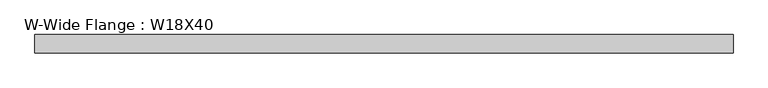
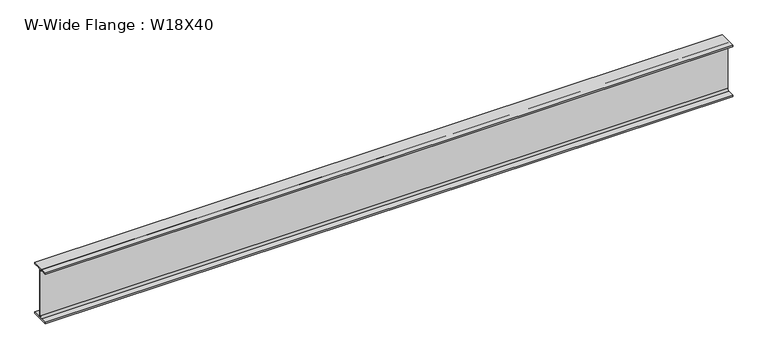
"""IFC4 building model written with IfcOpenShell, lengths in millimetres: beam geometry, W-Wide Flange : W18X40."""

import ifcopenshell
import ifcopenshell.guid

model = None  # the IFC model being written
_history = None  # IfcOwnerHistory: only IFC2X3 demands one
_inside = {}  # id of a spatial element -> (the spatial element, [elements in it])
_under = {}  # id of a project, library or spatial element -> (it, [spatial elements below it])
_declared = {}  # id of a project -> (the project, [libraries it declares])
_typed = {}  # id of a type object -> (the type object, [elements of that type])
_made_of = {}  # id of a material, layer set ... -> (it, [elements and type objects made of it])


def new_model(schema):
    """Start an empty IFC model of exactly this schema.

    Asked for "IFC4X3", IfcOpenShell would pick the latest addendum, in which some entities
    have other attributes; the version numbers below select the first issue.
    IFC2X3 requires an IfcOwnerHistory on every rooted entity: one is made here for all.
    """
    global model, _history
    if schema == "IFC4X3":
        model = ifcopenshell.file(schema_version=(4, 3, 0, 0))
    else:
        model = ifcopenshell.file(schema=schema)
    _inside.clear()
    _under.clear()
    _declared.clear()
    _typed.clear()
    _made_of.clear()
    _history = None
    if model.schema == "IFC2X3":
        org = make("IfcOrganization", Name="unknown")
        user = make(
            "IfcPersonAndOrganization",
            ThePerson=make("IfcPerson", FamilyName="unknown"),
            TheOrganization=org,
        )
        app = make(
            "IfcApplication",
            ApplicationDeveloper=org,
            Version="unknown",
            ApplicationFullName="unknown",
            ApplicationIdentifier="unknown",
        )
        _history = make(
            "IfcOwnerHistory",
            OwningUser=user,
            OwningApplication=app,
            ChangeAction="ADDED",
            CreationDate=0,
        )
    return model


def make(cls, **values):
    """One entity of the class cls with the attributes given. An attribute that is None is left unset."""
    return model.create_entity(
        cls, **{name: value for name, value in values.items() if value is not None}
    )


def rooted(cls, **values):
    """An entity with a GlobalId (a new one), such as an element, a storey or a relation."""
    return make(cls, GlobalId=ifcopenshell.guid.new(), OwnerHistory=_history, **values)


def si_unit(unit_type, name, prefix=None):
    """IfcSIUnit, for example si_unit("LENGTHUNIT", "METRE", prefix="MILLI")."""
    return make("IfcSIUnit", UnitType=unit_type, Prefix=prefix, Name=name)


def assignment(units):
    """IfcUnitAssignment: the units of a project."""
    return None if units is None else make("IfcUnitAssignment", Units=units)


def point(xyz):
    """IfcCartesianPoint."""
    return None if xyz is None else make("IfcCartesianPoint", Coordinates=xyz)


def direction(xyz):
    """IfcDirection."""
    return None if xyz is None else make("IfcDirection", DirectionRatios=xyz)


def frame(location, z_axis=None, x_axis=None):
    """IfcAxis2Placement3D, a coordinate frame: its origin and axes. An axis left out is left unset."""
    return make(
        "IfcAxis2Placement3D",
        Location=point(location),
        Axis=direction(z_axis),
        RefDirection=direction(x_axis),
    )


def frame_2d(location, x_axis=None):
    """IfcAxis2Placement2D, a coordinate frame in the plane: its origin and x axis."""
    return make(
        "IfcAxis2Placement2D", Location=point(location), RefDirection=direction(x_axis)
    )


def origin():
    """The frame at (0, 0, 0) with its axes left unset."""
    return frame((0.0, 0.0, 0.0))


def place(relative_to, where):
    """IfcLocalPlacement: puts the frame where relative to a parent placement (None: the world)."""
    return make(
        "IfcLocalPlacement", PlacementRelTo=relative_to, RelativePlacement=where
    )


def context(
    kind, dimensions, precision=None, world=None, true_north=None, identifier=None
):
    """IfcGeometricRepresentationContext, for example the 3D "Model" context."""
    return make(
        "IfcGeometricRepresentationContext",
        ContextIdentifier=identifier,
        ContextType=kind,
        CoordinateSpaceDimension=dimensions,
        Precision=precision,
        WorldCoordinateSystem=world,
        TrueNorth=true_north,
    )


def project(units=None, contexts=None):
    """IfcProject with its units and contexts."""
    return rooted(
        "IfcProject",
        Name="project",
        RepresentationContexts=contexts,
        UnitsInContext=assignment(units),
    )


def spatial(cls, under=None, at=None, **own):
    """A site, building, storey or space (cls), placed at a placement, below another one or the project."""
    s = rooted(cls, ObjectPlacement=at, **own)
    if under is not None:
        _under.setdefault(under.id(), (under, []))[1].append(s)
    return s


def polyline(points):
    """IfcPolyline through the points."""
    return make("IfcPolyline", Points=[point(p) for p in points])


def circle_curve(where, radius):
    """IfcCircle in the frame where."""
    return make("IfcCircle", Position=where, Radius=radius)


def trimmed(basis, trim1, trim2, sense, master):
    """IfcTrimmedCurve: the piece of a basis curve between two trims."""
    return make(
        "IfcTrimmedCurve",
        BasisCurve=basis,
        Trim1=trim1,
        Trim2=trim2,
        SenseAgreement=sense,
        MasterRepresentation=master,
    )


def segment(curve, same_sense, transition):
    """IfcCompositeCurveSegment."""
    return make(
        "IfcCompositeCurveSegment",
        Transition=transition,
        SameSense=same_sense,
        ParentCurve=curve,
    )


def composite_curve(segments, self_intersect=None):
    """IfcCompositeCurve: segments joined end to end."""
    return make("IfcCompositeCurve", Segments=segments, SelfIntersect=self_intersect)


def outline(outer, holes=None, kind="AREA"):
    """IfcArbitraryClosedProfileDef: a profile drawn as a closed curve; with holes, ...WithVoids."""
    if holes is None:
        return make("IfcArbitraryClosedProfileDef", ProfileType=kind, OuterCurve=outer)
    return make(
        "IfcArbitraryProfileDefWithVoids",
        ProfileType=kind,
        OuterCurve=outer,
        InnerCurves=holes,
    )


def extrude(swept, where, along, depth):
    """IfcExtrudedAreaSolid: the profile swept, set in the frame where, extruded along a direction by depth."""
    return make(
        "IfcExtrudedAreaSolid",
        SweptArea=swept,
        Position=where,
        ExtrudedDirection=direction(along),
        Depth=depth,
    )


def shape(context_of_items, identifier, shape_type, items):
    """IfcShapeRepresentation: the items that make up one representation, for example the "Body"."""
    return make(
        "IfcShapeRepresentation",
        ContextOfItems=context_of_items,
        RepresentationIdentifier=identifier,
        RepresentationType=shape_type,
        Items=items,
    )


def source(mapping_origin, context_of_items, identifier, shape_type, items):
    """IfcRepresentationMap: a shape defined once, which mapped items show again and again."""
    return make(
        "IfcRepresentationMap",
        MappingOrigin=mapping_origin,
        MappedRepresentation=shape(context_of_items, identifier, shape_type, items),
    )


def transform(
    local_origin,
    x_axis=None,
    y_axis=None,
    z_axis=None,
    scale=None,
    scale2=None,
    scale3=None,
    uniform=True,
):
    """IfcCartesianTransformationOperator3D, or its non-uniform kind. x_axis, y_axis, z_axis: its Axis1, 2, 3."""
    if uniform:
        return make(
            "IfcCartesianTransformationOperator3D",
            Axis1=direction(x_axis),
            Axis2=direction(y_axis),
            LocalOrigin=point(local_origin),
            Scale=scale,
            Axis3=direction(z_axis),
        )
    return make(
        "IfcCartesianTransformationOperator3DnonUniform",
        Axis1=direction(x_axis),
        Axis2=direction(y_axis),
        LocalOrigin=point(local_origin),
        Scale=scale,
        Axis3=direction(z_axis),
        Scale2=scale2,
        Scale3=scale3,
    )


def mapped(mapping_source, mapping_target):
    """IfcMappedItem: shows the shape of a source again, moved by a transform."""
    return make(
        "IfcMappedItem", MappingSource=mapping_source, MappingTarget=mapping_target
    )


def made_of(thing, what):
    """Note that an element or type object is made of a material, layer set ...; save() writes the relation."""
    if what is not None:
        _made_of.setdefault(what.id(), (what, []))[1].append(thing)
    return thing


def element(
    cls,
    number,
    at=None,
    inside=None,
    cuts=None,
    type_object=None,
    material=None,
    context=None,
    identifier="Body",
    shape_type=None,
    held_by="IfcProductDefinitionShape",
    body=None,
    shapes=None,
    **own,
):
    """One element of the class cls, such as IfcWall. Its Tag is "e" and its number.

    at: its placement. inside: the storey or other place that contains it. cuts: it is an
    opening in that element (IfcRelVoidsElement). A single representation is given by context,
    identifier, shape_type and body (its items); several are given by shapes. held_by: the class
    of the entity that holds the representations. save() writes the other relations.
    """
    e = rooted(cls, Tag="e%d" % number, ObjectPlacement=at, **own)
    if body is not None:
        shapes = [shape(context, identifier, shape_type, body)]
    if shapes is not None:
        e.Representation = make(held_by, Representations=shapes)
    if inside is not None:
        _inside.setdefault(inside.id(), (inside, []))[1].append(e)
    if cuts is not None:
        rooted(
            "IfcRelVoidsElement", RelatingBuildingElement=cuts, RelatedOpeningElement=e
        )
    if type_object is not None:
        _typed.setdefault(type_object.id(), (type_object, []))[1].append(e)
    return made_of(e, material)


def aggregate(whole, parts):
    """IfcRelAggregates: a whole, such as a stair, and the parts it consists of."""
    return rooted("IfcRelAggregates", RelatingObject=whole, RelatedObjects=parts)


def save(model, path):
    """Write the relations noted so far, then the file.

    IfcRelAggregates (storeys below a building ...), IfcRelContainedInSpatialStructure (elements
    in a storey), IfcRelDefinesByType, IfcRelAssociatesMaterial and IfcRelDeclares: one each for
    every whole, place, type object, material and project.
    """
    for whole, parts in _under.values():
        aggregate(whole, parts)
    for where, things in _inside.values():
        rooted(
            "IfcRelContainedInSpatialStructure",
            RelatedElements=things,
            RelatingStructure=where,
        )
    for kind, things in _typed.values():
        rooted("IfcRelDefinesByType", RelatedObjects=things, RelatingType=kind)
    for what, things in _made_of.values():
        rooted("IfcRelAssociatesMaterial", RelatedObjects=things, RelatingMaterial=what)
    for by, libraries in _declared.values():
        rooted("IfcRelDeclares", RelatingContext=by, RelatedDefinitions=libraries)
    model.write(path)


def w_wide_flange_w18x40_3d1222e0(model_context):
    return source(origin(), model_context, "Body", "SweptSolid", [
        extrude(outline(composite_curve([segment(polyline([(76.454, -213.995), (76.454, -227.33), (-76.454, -227.33), (-76.454, -213.995), (-20.828, -213.995)]), True, "CONTINUOUS"), segment(trimmed(circle_curve(frame_2d((-20.828, -197.1675)), 16.8275), [point((-20.828, -213.995))], [point((-4.0005, -197.1675))], True, "CARTESIAN"), True, "CONTINUOUS"), segment(polyline([(-4.0005, -197.1675), (-4.0005, 197.1675)]), True, "CONTINUOUS"), segment(trimmed(circle_curve(frame_2d((-20.828, 197.1675)), 16.8275), [point((-4.0005, 197.1675))], [point((-20.828, 213.995))], True, "CARTESIAN"), True, "CONTINUOUS"), segment(polyline([(-20.828, 213.995), (-76.454, 213.995), (-76.454, 227.33), (76.454, 227.33), (76.454, 213.995), (20.828, 213.995)]), True, "CONTINUOUS"), segment(trimmed(circle_curve(frame_2d((20.828, 197.1675)), 16.8275), [point((20.828, 213.995))], [point((4.0005, 197.1675))], True, "CARTESIAN"), True, "CONTINUOUS"), segment(polyline([(4.0005, 197.1675), (4.0005, -197.1675)]), True, "CONTINUOUS"), segment(trimmed(circle_curve(frame_2d((20.828, -197.1675)), 16.8275), [point((4.0005, -197.1675))], [point((20.828, -213.995))], True, "CARTESIAN"), True, "CONTINUOUS"), segment(polyline([(20.828, -213.995), (76.454, -213.995)]), True, "CONTINUOUS")], self_intersect=False)), frame((-2881.63, 0.0, 0.0), z_axis=(1.0, 0.0, 0.0), x_axis=(0.0, 1.0, 0.0)), (0.0, 0.0, 1.0), 5758.18),
    ])


if __name__ == "__main__":
    model = new_model("IFC4")
    model_context = context("Model", 3, world=origin())
    ifc_project = project(units=[si_unit("LENGTHUNIT", "METRE", prefix="MILLI")], contexts=[model_context])
    site = spatial("IfcSite", under=ifc_project)
    building = spatial("IfcBuilding", under=site)
    placement = place(None, origin())
    w_wide_flange_w18x40_shape = w_wide_flange_w18x40_3d1222e0(model_context)
    element("IfcBeam", 1, ObjectType="W-Wide Flange : W18X40", at=placement, inside=building, context=model_context, shape_type="MappedRepresentation", body=[
        mapped(w_wide_flange_w18x40_shape, transform((0.0, 0.0, 0.0), x_axis=(1.0, 0.0, 0.0), y_axis=(0.0, 1.0, 0.0), z_axis=(0.0, 0.0, 1.0))),
    ])
    save(model, "model.ifc")

# Revit data of these elements
# Type "W-Wide Flange : W18X40"
#   Assembly Code = "B10"
#   W = 40
#   Length [instance default] = 5' - 0"
#   bf = 0' - 6.02"
#   d = 1' - 5.9"
#   k = 0' - 1 3/16"
#   k2 = 0' - 0.6625"
#   tf = 0' - 0.525"
#   tw = 0' - 0.315"
#   A = 0.0819444 SF
#   Structural Material [instance default] = Steel ASTM A992
# Element 1 (IfcBeam, "W-Wide Flange : W18X40")
#   Materials on its faces: "Steel ASTM A992"
# Materials
#   "Steel ASTM A992": class "Metal", colour RGB 199 199 199, transparency 0, Description = "Structural steel 50ksi", Cost = 0
